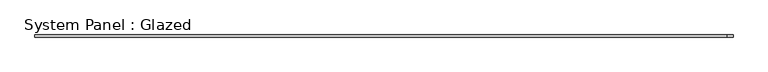
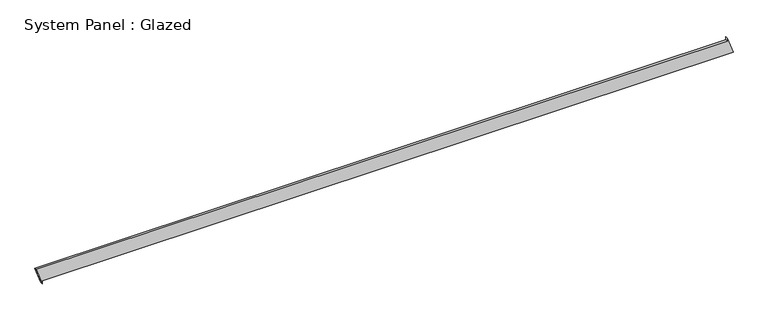
"""IFC4 building model written with IfcOpenShell, lengths in millimetres: plate geometry, System Panel : Glazed."""

from ifc_helpers import new_model, si_unit, frame, origin, place, context, project, spatial, polyline, outline, extrude, source, transform, mapped, element, save


def system_panel_glazed_dce2eccd(model_context):
    return source(origin(), model_context, "Body", "SweptSolid", [
        extrude(outline(polyline([(0.0, -3957.3100251), (35.3553391, -3957.3100251), (35.3553391, 4026.9402223), (234.465824, 3957.5777852), (199.110485, 3957.5782826), (198.9981604, -4026.9402223), (0.0, -3957.3100251)])), frame((0.0, -49.5, 0.0), z_axis=(0.0, 1.0, 0.0), x_axis=(0.0, 0.0, 1.0)), (0.0, 0.0, 1.0), 25.0),
    ])


if __name__ == "__main__":
    model = new_model("IFC4")
    model_context = context("Model", 3, world=origin())
    ifc_project = project(units=[si_unit("LENGTHUNIT", "METRE", prefix="MILLI")], contexts=[model_context])
    site = spatial("IfcSite", under=ifc_project)
    building = spatial("IfcBuilding", under=site)
    placement = place(None, origin())
    system_panel_glazed_shape = system_panel_glazed_dce2eccd(model_context)
    element("IfcPlate", 1, ObjectType="System Panel : Glazed", at=placement, inside=building, context=model_context, shape_type="MappedRepresentation", body=[
        mapped(system_panel_glazed_shape, transform((0.0, 0.0, 0.0), x_axis=(1.0, 0.0, 0.0), y_axis=(0.0, 1.0, 0.0), z_axis=(0.0, 0.0, 1.0))),
    ])
    save(model, "model.ifc")

# Revit data of these elements
# Element 1 (IfcPlate, "System Panel : Glazed")
#   Materials on its faces: "Glass"
# Materials
#   "Glass": class "Glass", colour RGB 218 227 224, transparency 0.85, Description = "Soda Lime Glass", Cost = 0
